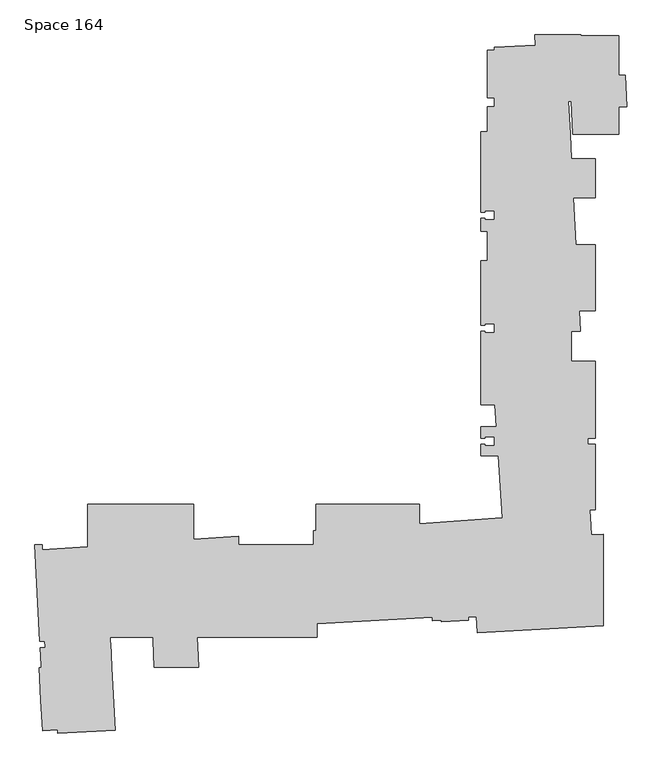
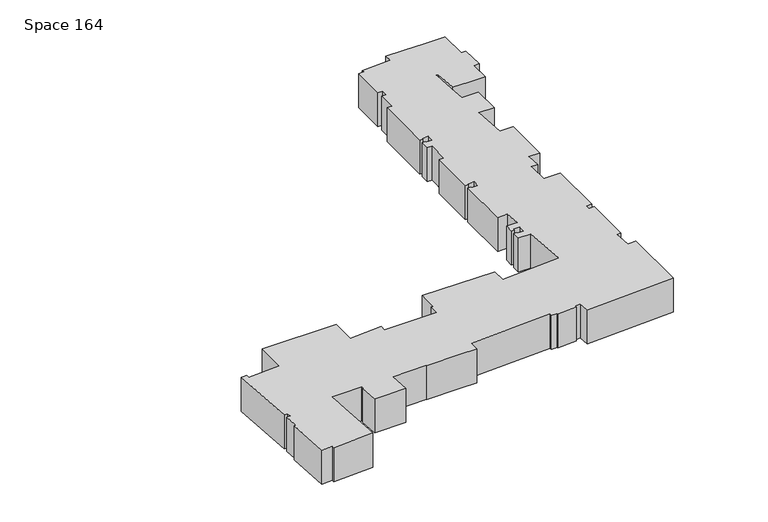
"""IFC4 building model written with IfcOpenShell, lengths in millimetres: proxy geometry, Space 164."""

from ifc_helpers import new_model, si_unit, origin, place, context, project, spatial, faceted_brep, source, transform, mapped, element, save


def space_164_15c8c7cc(model_context):
    return source(origin(), model_context, "Body", "Brep", [
        faceted_brep([(22026.6059655, -12784.934635, 0.0), (22026.6059655, -12422.984635, 0.0), (22026.6059655, -12422.984635, 3048.0), (22026.6059655, -12784.934635, 3048.0), (22483.8059655, -12784.934635, 0.0), (22483.8059655, -12784.934635, 3048.0), (22483.8059655, -16672.9333846, 0.0), (22483.8059655, -16672.9333846, 3048.0), (22156.2101931, -16690.1019516, 0.0), (22156.2101931, -16690.1019516, 3048.0), (22233.3115238, -18161.2829822, 0.0), (22177.9964598, -17105.8086856, 0.0), (22177.9964598, -17105.8086856, 3048.0), (22233.3115238, -18161.2829822, 3048.0), (22947.3559655, -18123.8614987, 0.0), (22483.8059655, -18148.1551247, 0.0), (22483.8059655, -18148.1551247, 3048.0), (22947.3559655, -18123.8614987, 3048.0), (22947.3559655, -23560.5623082, 0.0), (22947.3559655, -23560.5623082, 3048.0), (15462.7629947, -23952.8132046, 0.0), (15462.7629947, -23952.8132046, 3048.0), (15414.2423296, -23026.9837629, 0.0), (15438.3364955, -23486.727835, 0.0), (15438.3364955, -23486.727835, 3048.0), (15414.2423296, -23026.9837629, 3048.0), (14944.9863112, -23051.5764288, 0.0), (14944.9863112, -23051.5764288, 3048.0), (14954.2916443, -23229.1327601, 0.0), (14954.2916443, -23229.1327601, 3048.0), (13330.9194726, -23314.2100905, 0.0), (13330.9194726, -23314.2100905, 3048.0), (13326.9314727, -23238.11452, 0.0), (13326.9314727, -23238.11452, 3048.0), (12819.627669, -23264.7011857, 0.0), (12819.627669, -23264.7011857, 3048.0), (12808.9930027, -23061.7796643, 0.0), (12808.9930027, -23061.7796643, 3048.0), (5942.0559655, -23421.6605849, 0.0), (5942.0559655, -23421.6605849, 3048.0), (5942.0559655, -24227.634635, 0.0), (5942.0559655, -24227.634635, 3048.0), (1688.2936054, -24227.634635, 0.0), (1769.7735331, -24227.634635, 0.0), (4503.7809655, -24227.634635, 0.0), (4503.7809655, -24227.634635, 3048.0), (1769.7735331, -24227.634635, 3048.0), (1688.2936054, -24227.634635, 3048.0), (1688.2936054, -24237.159635, 0.0), (1688.2936054, -24237.159635, 3048.0), (-1166.2699748, -24237.159635, 0.0), (-1166.2699748, -24237.159635, 3048.0), (-1106.6703322, -25374.3885618, 0.0), (-1106.6703322, -25374.3885618, 3048.0), (-1116.1822785, -25374.8870618, 0.0), (-1116.1822785, -25374.8870618, 3048.0), (-1083.1261989, -26005.634635, 0.0), (-1083.1261989, -26005.634635, 3048.0), (-3709.2752449, -26005.634635, 0.0), (-3709.2752449, -26005.634635, 3048.0), (-3792.6318296, -24415.0962484, 0.0), (-3792.6318296, -24415.0962484, 3048.0), (-3783.1198833, -24414.5977484, 0.0), (-3783.1198833, -24414.5977484, 3048.0), (-3792.9182049, -24227.634635, 0.0), (-3792.9182049, -24227.634635, 3048.0), (-6336.4039637, -24227.634635, 0.0), (-6058.8520424, -24227.634635, 0.0), (-6058.8520424, -24227.634635, 3048.0), (-6336.4039637, -24227.634635, 3048.0), (-6319.6389015, -24547.5310773, 0.0), (-6323.7103915, -24469.8424208, 0.0), (-6323.7103915, -24469.8424208, 3048.0), (-6319.6389015, -24547.5310773, 3048.0), (-6310.1269552, -24547.0325773, 0.0), (-6310.1269552, -24547.0325773, 3048.0), (-6037.7797977, -29743.725916, 0.0), (-6233.6848605, -26005.634635, 0.0), (-6233.6848605, -26005.634635, 3048.0), (-6037.7797977, -29743.725916, 3048.0), (-9443.0565798, -29922.18891, 0.0), (-9443.0565798, -29922.18891, 3048.0), (-9452.8604128, -29735.1206324, 0.0), (-9452.8604128, -29735.1206324, 3048.0), (-10353.3246643, -29782.3119641, 0.0), (-10353.3246643, -29782.3119641, 3048.0), (-10548.7560157, -26053.259635, 0.0), (-10448.8704944, -27959.1889197, 0.0), (-10448.8704944, -27959.1889197, 3048.0), (-10548.7560157, -26053.259635, 3048.0), (-10421.9300647, -26046.6129686, 0.0), (-10421.9300647, -26046.6129686, 3048.0), (-10484.8878713, -24845.3064559, 0.0), (-10429.1798025, -25908.2797313, 0.0), (-10429.1798025, -25908.2797313, 3048.0), (-10484.8878713, -24845.3064559, 3048.0), (-10190.0175354, -24829.8529564, 0.0), (-10190.0175354, -24829.8529564, 3048.0), (-10208.9605348, -24468.3989963, 0.0), (-10208.9605348, -24468.3989963, 3048.0), (-10503.8308707, -24483.8524958, 0.0), (-10503.8308707, -24483.8524958, 3048.0), (-10804.9551147, -18738.059635, 0.0), (-10804.9551147, -18738.059635, 3048.0), (-10358.3940345, -18738.059635, 0.0), (-10358.3940345, -18738.059635, 3048.0), (-10358.3940345, -19055.4308203, 0.0), (-10358.3940345, -19055.4308203, 3048.0), (-7659.6440345, -18866.7158365, 0.0), (-7659.6440345, -18866.7158365, 3048.0), (-7659.6440345, -16350.459635, 0.0), (-7659.6440345, -16350.459635, 3048.0), (-1385.8440345, -16350.459635, 0.0), (-1385.8440345, -16350.459635, 3048.0), (-1385.8440345, -18428.0090038, 0.0), (-1385.8440345, -18428.0090038, 3048.0), (1306.5559655, -18239.7380553, 0.0), (1306.5559655, -18239.7380553, 3048.0), (1306.5559655, -18738.059635, 0.0), (1306.5559655, -18738.059635, 3048.0), (5751.5559655, -18738.059635, 0.0), (3059.1559655, -18738.059635, 0.0), (3059.1559655, -18738.059635, 3048.0), (5751.5559655, -18738.059635, 3048.0), (5751.5559655, -17928.9133762, 0.0), (5751.5559655, -17928.9133762, 3048.0), (5903.9559655, -17918.2565301, 0.0), (5903.9559655, -17918.2565301, 3048.0), (5903.9559655, -16350.459635, 0.0), (5903.9559655, -16350.459635, 3048.0), (12025.3559655, -16350.459635, 0.0), (12025.3559655, -16350.459635, 3048.0), (12025.3559655, -17490.2065434, 0.0), (12025.3559655, -17490.2065434, 3048.0), (16972.3711709, -17144.2775415, 0.0), (16972.3711709, -17144.2775415, 3048.0), (16715.7140446, -13473.909635, 0.0), (16715.7140446, -13473.909635, 3048.0), (15682.9559655, -13473.909635, 0.0), (15682.9559655, -13473.909635, 3048.0), (15682.9559655, -12788.109635, 0.0), (15682.9559655, -12788.109635, 3048.0), (15930.6059655, -12788.109635, 0.0), (15930.6059655, -12788.109635, 3048.0), (15930.6059655, -12877.009635, 0.0), (15930.6059655, -12877.009635, 3048.0), (16476.7059655, -12877.009635, 0.0), (16476.7059655, -12877.009635, 3048.0), (16476.7059655, -12330.909635, 0.0), (16476.7059655, -12330.909635, 3048.0), (15930.6059655, -12330.909635, 0.0), (15930.6059655, -12330.909635, 3048.0), (15930.6059655, -12419.809635, 0.0), (15930.6059655, -12419.809635, 3048.0), (15682.9559655, -12419.809635, 0.0), (15682.9559655, -12419.809635, 3048.0), (15682.9559655, -11734.009635, 0.0), (15682.9559655, -11734.009635, 3048.0), (16594.0483845, -11734.009635, 0.0), (16594.0483845, -11734.009635, 3048.0), (16503.021157, -10432.259635, 0.0), (16503.021157, -10432.259635, 3048.0), (15682.9559655, -10432.259635, 0.0), (15682.9559655, -10432.259635, 3048.0), (15682.9559655, -6082.509635, 0.0), (15682.9559655, -6082.509635, 3048.0), (15930.6059655, -6082.509635, 0.0), (15930.6059655, -6082.509635, 3048.0), (15930.6059655, -6171.409635, 0.0), (15930.6059655, -6171.409635, 3048.0), (16476.7059655, -6171.409635, 0.0), (16476.7059655, -6171.409635, 3048.0), (16476.7059655, -5625.309635, 0.0), (16476.7059655, -5625.309635, 3048.0), (15930.6059655, -5625.309635, 0.0), (15930.6059655, -5625.309635, 3048.0), (15930.6059655, -5714.209635, 0.0), (15930.6059655, -5714.209635, 3048.0), (15682.9559655, -5714.209635, 0.0), (15682.9559655, -5714.209635, 3048.0), (15682.9559655, -1897.859635, 0.0), (15682.9559655, -1897.859635, 3048.0), (16070.3059655, -1897.859635, 0.0), (16070.3059655, -1897.859635, 3048.0), (16070.3059655, -145.259635, 0.0), (16070.3059655, -145.259635, 3048.0), (15682.9559655, -145.259635, 0.0), (15682.9559655, -145.259635, 3048.0), (15682.9559655, 623.090365, 0.0), (15682.9559655, 623.090365, 3048.0), (15930.6059655, 623.090365, 0.0), (15930.6059655, 623.090365, 3048.0), (15930.6059655, 534.190365, 0.0), (15930.6059655, 534.190365, 3048.0), (16476.7059655, 534.190365, 0.0), (16476.7059655, 534.190365, 3048.0), (16476.7059655, 1080.290365, 0.0), (16476.7059655, 1080.290365, 3048.0), (15930.6059655, 1080.290365, 0.0), (15930.6059655, 1080.290365, 3048.0), (15930.6059655, 991.390365, 0.0), (15930.6059655, 991.390365, 3048.0), (15682.9559655, 991.390365, 0.0), (15682.9559655, 991.390365, 3048.0), (15682.9559655, 5772.940365, 0.0), (15682.9559655, 5772.940365, 3048.0), (16070.3059655, 5772.940365, 0.0), (16070.3059655, 5772.940365, 3048.0), (16070.3059655, 7239.790365, 0.0), (16070.3059655, 7175.680765, 0.0), (16070.3059655, 7175.680765, 3048.0), (16070.3059655, 7239.790365, 3048.0), (16476.7059655, 7239.790365, 0.0), (16476.7059655, 7239.790365, 3048.0), (16476.7059655, 7785.890365, 0.0), (16476.7059655, 7785.890365, 3048.0), (16070.3059655, 7785.890365, 0.0), (16070.3059655, 7785.890365, 3048.0), (16070.3059655, 10592.590365, 0.0), (16070.3059655, 10528.480765, 0.0), (16070.3059655, 7849.999965, 0.0), (16070.3059655, 7849.999965, 3048.0), (16070.3059655, 10528.480765, 3048.0), (16070.3059655, 10592.590365, 3048.0), (16476.7059655, 10592.590365, 0.0), (16476.7059655, 10592.590365, 3048.0), (16476.7059655, 10776.6183634, 0.0), (16476.7059655, 10776.6183634, 3048.0), (18930.2144031, 10905.2012921, 0.0), (16481.4421221, 10776.8665749, 0.0), (16481.4421221, 10776.8665749, 3048.0), (18930.2144031, 10905.2012921, 3048.0), (18898.3431848, 11513.340365, 0.0), (18898.3431848, 11513.340365, 3048.0), (21629.7309655, 11513.340365, 0.0), (21629.7309655, 11513.340365, 3048.0), (21629.7309655, 11465.715365, 0.0), (21629.7309655, 11465.715365, 3048.0), (23880.8059655, 11465.715365, 0.0), (23804.6059655, 11465.715365, 0.0), (23804.6059655, 11465.715365, 3048.0), (23880.8059655, 11465.715365, 3048.0), (23880.8059655, 9122.565365, 0.0), (23880.8059655, 9122.565365, 3048.0), (24256.4516722, 9122.565365, 0.0), (24256.4516722, 9122.565365, 3048.0), (24354.2917553, 7255.665365, 0.0), (24354.2917553, 7255.665365, 3048.0), (23880.8059655, 7255.665365, 0.0), (23880.8059655, 7255.665365, 3048.0), (23880.8059655, 5617.365365, 0.0), (23880.8059655, 5617.365365, 3048.0), (21155.6313011, 5617.365365, 0.0), (22483.8059655, 5617.365365, 0.0), (22483.8059655, 5617.365365, 3048.0), (21155.6313011, 5617.365365, 3048.0), (21053.17681, 7572.3135147, 0.0), (21053.17681, 7572.3135147, 3048.0), (20885.132425, 7563.5066816, 0.0), (20885.132425, 7563.5066816, 3048.0), (21063.5005365, 4160.040365, 0.0), (20987.1253696, 5617.365365, 0.0), (20987.1253696, 5617.365365, 3048.0), (21063.5005365, 4160.040365, 3048.0), (22483.8059655, 4160.040365, 0.0), (22483.8059655, 4160.040365, 3048.0), (22483.8059655, 1848.640365, 0.0), (22483.8059655, 1848.640365, 3048.0), (21184.6358776, 1848.640365, 0.0), (21184.6358776, 1848.640365, 3048.0), (21330.3976341, -932.659635, 0.0), (21330.3976341, -932.659635, 3048.0), (22483.8059655, -932.659635, 0.0), (22483.8059655, -932.659635, 3048.0), (22483.8059655, -4856.959635, 0.0), (22483.8059655, -4856.959635, 3048.0), (21536.0614823, -4856.959635, 0.0), (21536.0614823, -4856.959635, 3048.0), (21599.291468, -6063.459635, 0.0), (21599.291468, -6063.459635, 3048.0), (21069.1360612, -6063.459635, 0.0), (21069.1360612, -6063.459635, 3048.0), (21069.1360612, -7847.809635, 0.0), (21069.1360612, -7847.809635, 3048.0), (22483.8059655, -7847.809635, 0.0), (22483.8059655, -7847.809635, 3048.0), (22483.8059655, -12422.984635, 0.0), (22483.8059655, -12422.984635, 3048.0)], [[[0, 1, 2, 3]], [[4, 0, 3, 5]], [[6, 4, 5, 7]], [[8, 6, 7, 9]], [[10, 11, 8, 9, 12, 13]], [[14, 15, 10, 13, 16, 17]], [[18, 14, 17, 19]], [[20, 18, 19, 21]], [[22, 23, 20, 21, 24, 25]], [[26, 22, 25, 27]], [[28, 26, 27, 29]], [[30, 28, 29, 31]], [[32, 30, 31, 33]], [[34, 32, 33, 35]], [[36, 34, 35, 37]], [[38, 36, 37, 39]], [[40, 38, 39, 41]], [[42, 43, 44, 40, 41, 45, 46, 47]], [[48, 42, 47, 49]], [[50, 48, 49, 51]], [[52, 50, 51, 53]], [[54, 52, 53, 55]], [[56, 54, 55, 57]], [[58, 56, 57, 59]], [[60, 58, 59, 61]], [[62, 60, 61, 63]], [[64, 62, 63, 65]], [[66, 67, 64, 65, 68, 69]], [[70, 71, 66, 69, 72, 73]], [[74, 70, 73, 75]], [[76, 77, 74, 75, 78, 79]], [[80, 76, 79, 81]], [[82, 80, 81, 83]], [[84, 82, 83, 85]], [[86, 87, 84, 85, 88, 89]], [[90, 86, 89, 91]], [[92, 93, 90, 91, 94, 95]], [[96, 92, 95, 97]], [[98, 96, 97, 99]], [[100, 98, 99, 101]], [[102, 100, 101, 103]], [[104, 102, 103, 105]], [[106, 104, 105, 107]], [[108, 106, 107, 109]], [[110, 108, 109, 111]], [[112, 110, 111, 113]], [[114, 112, 113, 115]], [[116, 114, 115, 117]], [[118, 116, 117, 119]], [[120, 121, 118, 119, 122, 123]], [[124, 120, 123, 125]], [[126, 124, 125, 127]], [[128, 126, 127, 129]], [[130, 128, 129, 131]], [[132, 130, 131, 133]], [[134, 132, 133, 135]], [[136, 134, 135, 137]], [[138, 136, 137, 139]], [[140, 138, 139, 141]], [[142, 140, 141, 143]], [[144, 142, 143, 145]], [[146, 144, 145, 147]], [[148, 146, 147, 149]], [[150, 148, 149, 151]], [[152, 150, 151, 153]], [[154, 152, 153, 155]], [[156, 154, 155, 157]], [[158, 156, 157, 159]], [[160, 158, 159, 161]], [[162, 160, 161, 163]], [[164, 162, 163, 165]], [[166, 164, 165, 167]], [[168, 166, 167, 169]], [[170, 168, 169, 171]], [[172, 170, 171, 173]], [[174, 172, 173, 175]], [[176, 174, 175, 177]], [[178, 176, 177, 179]], [[180, 178, 179, 181]], [[182, 180, 181, 183]], [[184, 182, 183, 185]], [[186, 184, 185, 187]], [[188, 186, 187, 189]], [[190, 188, 189, 191]], [[192, 190, 191, 193]], [[194, 192, 193, 195]], [[196, 194, 195, 197]], [[198, 196, 197, 199]], [[200, 198, 199, 201]], [[202, 200, 201, 203]], [[204, 202, 203, 205]], [[206, 204, 205, 207]], [[208, 209, 206, 207, 210, 211]], [[212, 208, 211, 213]], [[214, 212, 213, 215]], [[216, 214, 215, 217]], [[218, 219, 220, 216, 217, 221, 222, 223]], [[224, 218, 223, 225]], [[226, 224, 225, 227]], [[228, 229, 226, 227, 230, 231]], [[232, 228, 231, 233]], [[234, 232, 233, 235]], [[236, 234, 235, 237]], [[238, 239, 236, 237, 240, 241]], [[242, 238, 241, 243]], [[244, 242, 243, 245]], [[246, 244, 245, 247]], [[248, 246, 247, 249]], [[250, 248, 249, 251]], [[252, 253, 250, 251, 254, 255]], [[256, 252, 255, 257]], [[258, 256, 257, 259]], [[260, 261, 258, 259, 262, 263]], [[264, 260, 263, 265]], [[266, 264, 265, 267]], [[268, 266, 267, 269]], [[270, 268, 269, 271]], [[272, 270, 271, 273]], [[274, 272, 273, 275]], [[276, 274, 275, 277]], [[278, 276, 277, 279]], [[280, 278, 279, 281]], [[282, 280, 281, 283]], [[284, 282, 283, 285]], [[286, 284, 285, 287]], [[1, 286, 287, 2]], [[2, 287, 285, 283, 281, 279, 277, 275, 273, 271, 269, 267, 265, 263, 262, 259, 257, 255, 254, 251, 249, 247, 245, 243, 241, 240, 237, 235, 233, 231, 230, 227, 225, 223, 222, 221, 217, 215, 213, 211, 210, 207, 205, 203, 201, 199, 197, 195, 193, 191, 189, 187, 185, 183, 181, 179, 177, 175, 173, 171, 169, 167, 165, 163, 161, 159, 157, 155, 153, 151, 149, 147, 145, 143, 141, 139, 137, 135, 133, 131, 129, 127, 125, 123, 122, 119, 117, 115, 113, 111, 109, 107, 105, 103, 101, 99, 97, 95, 94, 91, 89, 88, 85, 83, 81, 79, 78, 75, 73, 72, 69, 68, 65, 63, 61, 59, 57, 55, 53, 51, 49, 47, 46, 45, 41, 39, 37, 35, 33, 31, 29, 27, 25, 24, 21, 19, 17, 16, 13, 12, 9, 7, 5, 3]], [[286, 1, 0, 4, 6, 8, 11, 10, 15, 14, 18, 20, 23, 22, 26, 28, 30, 32, 34, 36, 38, 40, 44, 43, 42, 48, 50, 52, 54, 56, 58, 60, 62, 64, 67, 66, 71, 70, 74, 77, 76, 80, 82, 84, 87, 86, 90, 93, 92, 96, 98, 100, 102, 104, 106, 108, 110, 112, 114, 116, 118, 121, 120, 124, 126, 128, 130, 132, 134, 136, 138, 140, 142, 144, 146, 148, 150, 152, 154, 156, 158, 160, 162, 164, 166, 168, 170, 172, 174, 176, 178, 180, 182, 184, 186, 188, 190, 192, 194, 196, 198, 200, 202, 204, 206, 209, 208, 212, 214, 216, 220, 219, 218, 224, 226, 229, 228, 232, 234, 236, 239, 238, 242, 244, 246, 248, 250, 253, 252, 256, 258, 261, 260, 264, 266, 268, 270, 272, 274, 276, 278, 280, 282, 284]]]),
    ])


if __name__ == "__main__":
    model = new_model("IFC4")
    model_context = context("Model", 3, world=origin())
    ifc_project = project(units=[si_unit("LENGTHUNIT", "METRE", prefix="MILLI")], contexts=[model_context])
    site = spatial("IfcSite", under=ifc_project)
    building = spatial("IfcBuilding", under=site)
    placement = place(None, origin())
    space_164_shape = space_164_15c8c7cc(model_context)
    element("IfcBuildingElementProxy", 1, Name="Space 164", ObjectType="Space 164", at=placement, inside=building, context=model_context, shape_type="MappedRepresentation", body=[
        mapped(space_164_shape, transform((0.0, 0.0, 0.0), x_axis=(1.0, 0.0, 0.0), y_axis=(0.0, 1.0, 0.0), z_axis=(0.0, 0.0, 1.0))),
    ])
    save(model, "model.ifc")

# Revit data of these elements
# Element 1 (IfcBuildingElementProxy, "Space 164")
#   Materials on its faces: "Render Material 255-255-255"
# Materials
#   "Render Material 255-255-255": class "Unassigned", colour RGB 255 255 255, transparency 0
